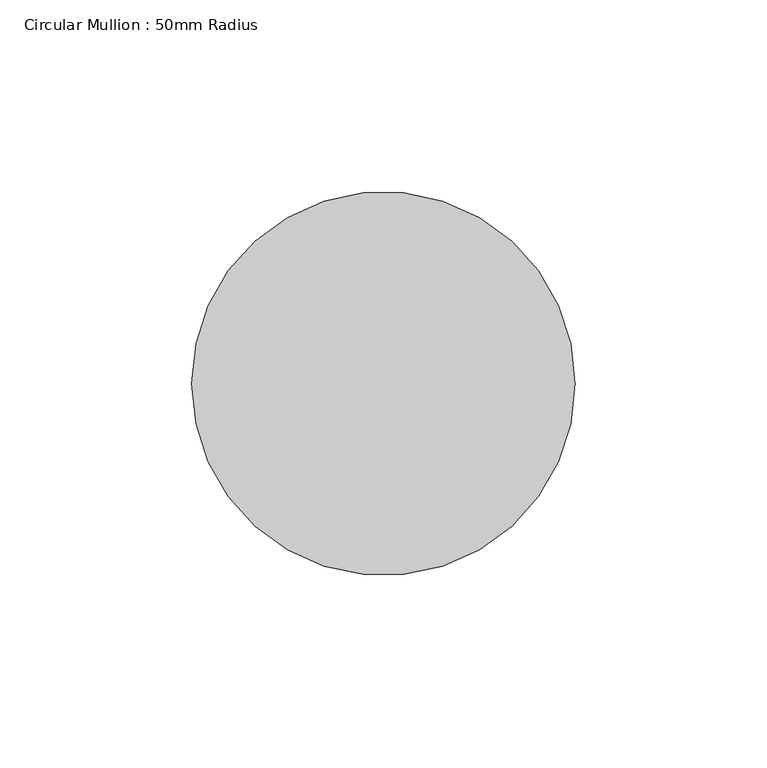
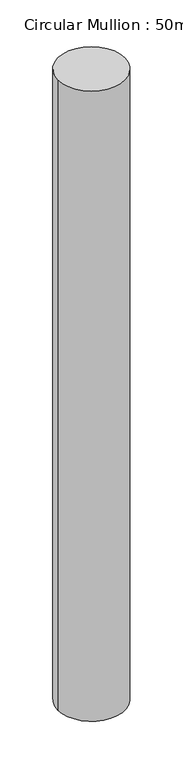
"""IFC4 building model written with IfcOpenShell, lengths in millimetres: member geometry, Circular Mullion : 50mm Radius."""

from ifc_helpers import new_model, si_unit, point, frame, origin, origin_2d, place, context, project, spatial, circle_curve, trimmed, segment, composite_curve, outline, extrude, source, transform, mapped, element, save


def circular_mullion_50mm_radius_7fba7e34(model_context):
    return source(origin(), model_context, "Body", "SweptSolid", [
        extrude(outline(composite_curve([segment(trimmed(circle_curve(origin_2d(), 50.0), [point((50.0, 0.0))], [point((-50.0, 0.0))], False, "CARTESIAN"), True, "CONTINUOUS"), segment(trimmed(circle_curve(origin_2d(), 50.0), [point((-50.0, 0.0))], [point((50.0, 0.0))], False, "CARTESIAN"), True, "CONTINUOUS")], self_intersect=False)), frame((0.0, 0.0, -995.7633594), z_axis=(0.0, 0.0, 1.0), x_axis=(1.0, 0.0, 0.0)), (0.0, 0.0, 1.0), 995.7633594),
    ])


if __name__ == "__main__":
    model = new_model("IFC4")
    model_context = context("Model", 3, world=origin())
    ifc_project = project(units=[si_unit("LENGTHUNIT", "METRE", prefix="MILLI")], contexts=[model_context])
    site = spatial("IfcSite", under=ifc_project)
    building = spatial("IfcBuilding", under=site)
    placement = place(None, origin())
    circular_mullion_50mm_radius_shape = circular_mullion_50mm_radius_7fba7e34(model_context)
    element("IfcMember", 1, ObjectType="Circular Mullion : 50mm Radius", at=placement, inside=building, context=model_context, shape_type="MappedRepresentation", body=[
        mapped(circular_mullion_50mm_radius_shape, transform((0.0, 0.0, 0.0), x_axis=(1.0, 0.0, 0.0), y_axis=(0.0, 1.0, 0.0), z_axis=(0.0, 0.0, 1.0))),
    ])
    save(model, "model.ifc")

# Revit data of these elements
# Type "Circular Mullion : 50mm Radius"
#   built-in parameter 1007350 = 0.164042 (stored number, unit not read)
# Element 1 (IfcMember, "Circular Mullion : 50mm Radius")
#   Materials on its faces: "Aluminium"
# Materials
#   "Aluminium": class "Metal", colour RGB 247 247 247, transparency 0, Description = "Aluminium 6061", Cost = 0
